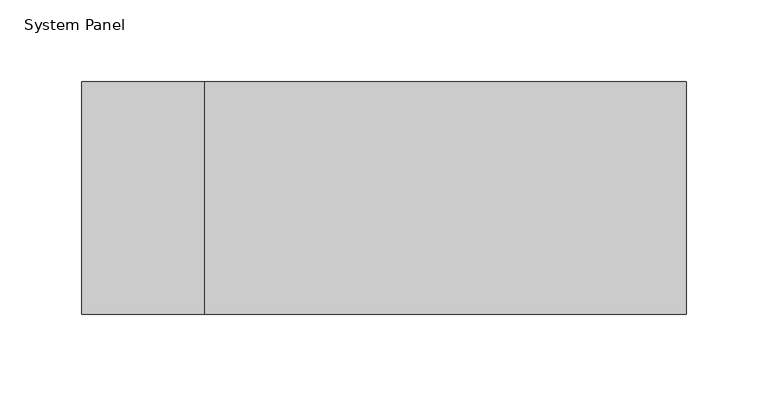
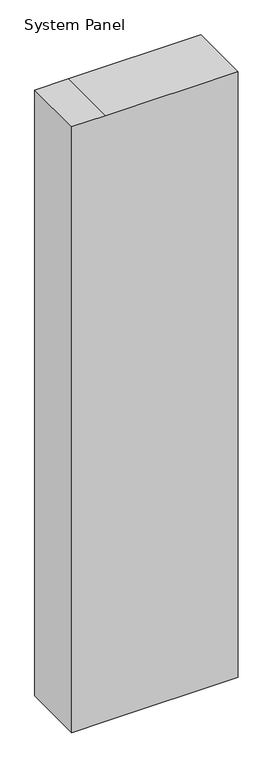
"""IFC4 building model written with IfcOpenShell, lengths in millimetres: plate geometry, System Panel : NLRS_21_CWP_hsb-vulling minerale wol 142 _gen_rsf."""

import ifcopenshell
import ifcopenshell.guid

model = None  # the IFC model being written
_history = None  # IfcOwnerHistory: only IFC2X3 demands one
_inside = {}  # id of a spatial element -> (the spatial element, [elements in it])
_under = {}  # id of a project, library or spatial element -> (it, [spatial elements below it])
_declared = {}  # id of a project -> (the project, [libraries it declares])
_typed = {}  # id of a type object -> (the type object, [elements of that type])
_made_of = {}  # id of a material, layer set ... -> (it, [elements and type objects made of it])


def new_model(schema):
    """Start an empty IFC model of exactly this schema.

    Asked for "IFC4X3", IfcOpenShell would pick the latest addendum, in which some entities
    have other attributes; the version numbers below select the first issue.
    IFC2X3 requires an IfcOwnerHistory on every rooted entity: one is made here for all.
    """
    global model, _history
    if schema == "IFC4X3":
        model = ifcopenshell.file(schema_version=(4, 3, 0, 0))
    else:
        model = ifcopenshell.file(schema=schema)
    _inside.clear()
    _under.clear()
    _declared.clear()
    _typed.clear()
    _made_of.clear()
    _history = None
    if model.schema == "IFC2X3":
        org = make("IfcOrganization", Name="unknown")
        user = make(
            "IfcPersonAndOrganization",
            ThePerson=make("IfcPerson", FamilyName="unknown"),
            TheOrganization=org,
        )
        app = make(
            "IfcApplication",
            ApplicationDeveloper=org,
            Version="unknown",
            ApplicationFullName="unknown",
            ApplicationIdentifier="unknown",
        )
        _history = make(
            "IfcOwnerHistory",
            OwningUser=user,
            OwningApplication=app,
            ChangeAction="ADDED",
            CreationDate=0,
        )
    return model


def make(cls, **values):
    """One entity of the class cls with the attributes given. An attribute that is None is left unset."""
    return model.create_entity(
        cls, **{name: value for name, value in values.items() if value is not None}
    )


def rooted(cls, **values):
    """An entity with a GlobalId (a new one), such as an element, a storey or a relation."""
    return make(cls, GlobalId=ifcopenshell.guid.new(), OwnerHistory=_history, **values)


def si_unit(unit_type, name, prefix=None):
    """IfcSIUnit, for example si_unit("LENGTHUNIT", "METRE", prefix="MILLI")."""
    return make("IfcSIUnit", UnitType=unit_type, Prefix=prefix, Name=name)


def assignment(units):
    """IfcUnitAssignment: the units of a project."""
    return None if units is None else make("IfcUnitAssignment", Units=units)


def point(xyz):
    """IfcCartesianPoint."""
    return None if xyz is None else make("IfcCartesianPoint", Coordinates=xyz)


def direction(xyz):
    """IfcDirection."""
    return None if xyz is None else make("IfcDirection", DirectionRatios=xyz)


def frame(location, z_axis=None, x_axis=None):
    """IfcAxis2Placement3D, a coordinate frame: its origin and axes. An axis left out is left unset."""
    return make(
        "IfcAxis2Placement3D",
        Location=point(location),
        Axis=direction(z_axis),
        RefDirection=direction(x_axis),
    )


def origin():
    """The frame at (0, 0, 0) with its axes left unset."""
    return frame((0.0, 0.0, 0.0))


def place(relative_to, where):
    """IfcLocalPlacement: puts the frame where relative to a parent placement (None: the world)."""
    return make(
        "IfcLocalPlacement", PlacementRelTo=relative_to, RelativePlacement=where
    )


def context(
    kind, dimensions, precision=None, world=None, true_north=None, identifier=None
):
    """IfcGeometricRepresentationContext, for example the 3D "Model" context."""
    return make(
        "IfcGeometricRepresentationContext",
        ContextIdentifier=identifier,
        ContextType=kind,
        CoordinateSpaceDimension=dimensions,
        Precision=precision,
        WorldCoordinateSystem=world,
        TrueNorth=true_north,
    )


def project(units=None, contexts=None):
    """IfcProject with its units and contexts."""
    return rooted(
        "IfcProject",
        Name="project",
        RepresentationContexts=contexts,
        UnitsInContext=assignment(units),
    )


def spatial(cls, under=None, at=None, **own):
    """A site, building, storey or space (cls), placed at a placement, below another one or the project."""
    s = rooted(cls, ObjectPlacement=at, **own)
    if under is not None:
        _under.setdefault(under.id(), (under, []))[1].append(s)
    return s


def polyline(points):
    """IfcPolyline through the points."""
    return make("IfcPolyline", Points=[point(p) for p in points])


def outline(outer, holes=None, kind="AREA"):
    """IfcArbitraryClosedProfileDef: a profile drawn as a closed curve; with holes, ...WithVoids."""
    if holes is None:
        return make("IfcArbitraryClosedProfileDef", ProfileType=kind, OuterCurve=outer)
    return make(
        "IfcArbitraryProfileDefWithVoids",
        ProfileType=kind,
        OuterCurve=outer,
        InnerCurves=holes,
    )


def extrude(swept, where, along, depth):
    """IfcExtrudedAreaSolid: the profile swept, set in the frame where, extruded along a direction by depth."""
    return make(
        "IfcExtrudedAreaSolid",
        SweptArea=swept,
        Position=where,
        ExtrudedDirection=direction(along),
        Depth=depth,
    )


def shape(context_of_items, identifier, shape_type, items):
    """IfcShapeRepresentation: the items that make up one representation, for example the "Body"."""
    return make(
        "IfcShapeRepresentation",
        ContextOfItems=context_of_items,
        RepresentationIdentifier=identifier,
        RepresentationType=shape_type,
        Items=items,
    )


def source(mapping_origin, context_of_items, identifier, shape_type, items):
    """IfcRepresentationMap: a shape defined once, which mapped items show again and again."""
    return make(
        "IfcRepresentationMap",
        MappingOrigin=mapping_origin,
        MappedRepresentation=shape(context_of_items, identifier, shape_type, items),
    )


def transform(
    local_origin,
    x_axis=None,
    y_axis=None,
    z_axis=None,
    scale=None,
    scale2=None,
    scale3=None,
    uniform=True,
):
    """IfcCartesianTransformationOperator3D, or its non-uniform kind. x_axis, y_axis, z_axis: its Axis1, 2, 3."""
    if uniform:
        return make(
            "IfcCartesianTransformationOperator3D",
            Axis1=direction(x_axis),
            Axis2=direction(y_axis),
            LocalOrigin=point(local_origin),
            Scale=scale,
            Axis3=direction(z_axis),
        )
    return make(
        "IfcCartesianTransformationOperator3DnonUniform",
        Axis1=direction(x_axis),
        Axis2=direction(y_axis),
        LocalOrigin=point(local_origin),
        Scale=scale,
        Axis3=direction(z_axis),
        Scale2=scale2,
        Scale3=scale3,
    )


def mapped(mapping_source, mapping_target):
    """IfcMappedItem: shows the shape of a source again, moved by a transform."""
    return make(
        "IfcMappedItem", MappingSource=mapping_source, MappingTarget=mapping_target
    )


def made_of(thing, what):
    """Note that an element or type object is made of a material, layer set ...; save() writes the relation."""
    if what is not None:
        _made_of.setdefault(what.id(), (what, []))[1].append(thing)
    return thing


def element(
    cls,
    number,
    at=None,
    inside=None,
    cuts=None,
    type_object=None,
    material=None,
    context=None,
    identifier="Body",
    shape_type=None,
    held_by="IfcProductDefinitionShape",
    body=None,
    shapes=None,
    **own,
):
    """One element of the class cls, such as IfcWall. Its Tag is "e" and its number.

    at: its placement. inside: the storey or other place that contains it. cuts: it is an
    opening in that element (IfcRelVoidsElement). A single representation is given by context,
    identifier, shape_type and body (its items); several are given by shapes. held_by: the class
    of the entity that holds the representations. save() writes the other relations.
    """
    e = rooted(cls, Tag="e%d" % number, ObjectPlacement=at, **own)
    if body is not None:
        shapes = [shape(context, identifier, shape_type, body)]
    if shapes is not None:
        e.Representation = make(held_by, Representations=shapes)
    if inside is not None:
        _inside.setdefault(inside.id(), (inside, []))[1].append(e)
    if cuts is not None:
        rooted(
            "IfcRelVoidsElement", RelatingBuildingElement=cuts, RelatedOpeningElement=e
        )
    if type_object is not None:
        _typed.setdefault(type_object.id(), (type_object, []))[1].append(e)
    return made_of(e, material)


def aggregate(whole, parts):
    """IfcRelAggregates: a whole, such as a stair, and the parts it consists of."""
    return rooted("IfcRelAggregates", RelatingObject=whole, RelatedObjects=parts)


def save(model, path):
    """Write the relations noted so far, then the file.

    IfcRelAggregates (storeys below a building ...), IfcRelContainedInSpatialStructure (elements
    in a storey), IfcRelDefinesByType, IfcRelAssociatesMaterial and IfcRelDeclares: one each for
    every whole, place, type object, material and project.
    """
    for whole, parts in _under.values():
        aggregate(whole, parts)
    for where, things in _inside.values():
        rooted(
            "IfcRelContainedInSpatialStructure",
            RelatedElements=things,
            RelatingStructure=where,
        )
    for kind, things in _typed.values():
        rooted("IfcRelDefinesByType", RelatedObjects=things, RelatingType=kind)
    for what, things in _made_of.values():
        rooted("IfcRelAssociatesMaterial", RelatedObjects=things, RelatingMaterial=what)
    for by, libraries in _declared.values():
        rooted("IfcRelDeclares", RelatingContext=by, RelatedDefinitions=libraries)
    model.write(path)


def system_panel_a8f59ee8(model_context):
    return source(origin(), model_context, "Body", "SweptSolid", [
        extrude(outline(polyline([(0.0, -184.5), (0.0, -109.3441061), (0.0, 184.5), (1421.0, 184.5), (1421.0, -109.3441061), (1421.0, -184.5), (0.0, -184.5)])), frame((0.0, -71.0, 0.0), z_axis=(0.0, 1.0, 0.0), x_axis=(0.0, 0.0, 1.0)), (0.0, 0.0, 1.0), 142.0),
    ])


if __name__ == "__main__":
    model = new_model("IFC4")
    model_context = context("Model", 3, world=origin())
    ifc_project = project(units=[si_unit("LENGTHUNIT", "METRE", prefix="MILLI")], contexts=[model_context])
    site = spatial("IfcSite", under=ifc_project)
    building = spatial("IfcBuilding", under=site)
    placement = place(None, origin())
    system_panel_shape = system_panel_a8f59ee8(model_context)
    element("IfcPlate", 1, ObjectType="System Panel : NLRS_21_CWP_hsb-vulling minerale wol 142 _gen_rsf", at=placement, inside=building, context=model_context, shape_type="MappedRepresentation", body=[
        mapped(system_panel_shape, transform((0.0, 0.0, 0.0), x_axis=(1.0, 0.0, 0.0), y_axis=(0.0, 1.0, 0.0), z_axis=(0.0, 0.0, 1.0))),
    ])
    save(model, "model.ifc")

# Revit data of these elements
# Type "System Panel : NLRS_21_CWP_hsb-vulling minerale wol 142 _gen_rsf"
#   Export Type to IFC As = "IfcWall"
#   Type IfcGUID = "07M7mRoiH1CR8m_RSKIwpC"
#   Assembly Code = "21.23"
# Element 1 (IfcPlate, "System Panel : NLRS_21_CWP_hsb-vulling minerale wol 142 _gen_rsf")
#   Materials on its faces: "NLRS_m1_isolatie minerale wol_gen_rsf"
# Materials
#   "NLRS_m1_isolatie minerale wol_gen_rsf": class "M - Anorganische materialen", colour RGB 200 200 140, transparency 0, Keynote = "m1", Manufacturer = "Revit Standards Foundation", URL = "www.revitstandards.org", Description = "isolatie minerale wol", Cost = 0
